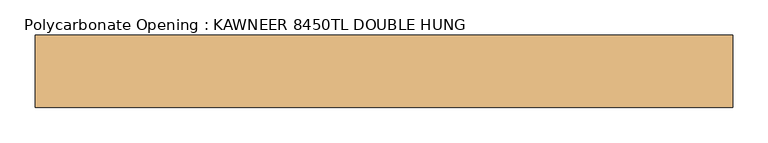
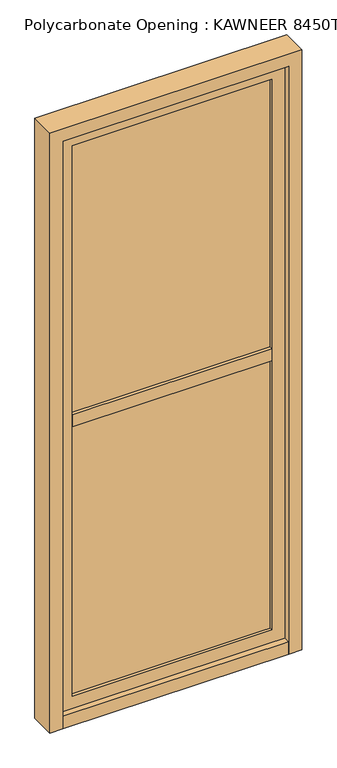
"""IFC4 building model written with IfcOpenShell, lengths in millimetres: door geometry, Polycarbonate Opening : KAWNEER 8450TL DOUBLE HUNG."""

from ifc_helpers import new_model, si_unit, frame, origin, origin_with_axes, place, context, project, spatial, polyline, outline, extrude, source, transform, mapped, element, save


def polycarbonate_opening_kawneer_8450tl_double_hung_34cef571(model_context):
    return source(origin(), model_context, "Body", "SweptSolid", [
        extrude(outline(polyline([(440.1908884, 12.7), (440.1908884, -12.7), (-440.1908884, -12.7), (-440.1908884, 12.7), (440.1908884, 12.7)])), frame((0.0, 0.0, 50.8), z_axis=(0.0, 0.0, 1.0), x_axis=(1.0, 0.0, 0.0)), (0.0, 0.0, 1.0), 2371.4648118),
        extrude(outline(polyline([(2422.2648118, -440.1908884), (0.0, -440.1908884), (0.0, 440.1908884), (2422.2648118, 440.1908884), (2422.2648118, -440.1908884)]), holes=[polyline([(101.6, 389.3908884), (101.6, -389.3908884), (2371.4648118, -389.3908884), (2371.4648118, 389.3908884), (101.6, 389.3908884)])]), frame((0.0, -25.4, 0.0), z_axis=(0.0, 1.0, 0.0), x_axis=(0.0, 0.0, 1.0)), (0.0, 0.0, 1.0), 50.8),
        extrude(outline(polyline([(2473.0648118, 490.9908884), (2473.0648118, -490.9908884), (0.0, -490.9908884), (0.0, -440.1908884), (2422.2648118, -440.1908884), (2422.2648118, 440.1908884), (0.0, 440.1908884), (0.0, 490.9908884), (2473.0648118, 490.9908884)])), frame((0.0, -50.8, 0.0), z_axis=(0.0, 1.0, 0.0), x_axis=(0.0, 0.0, 1.0)), (0.0, 0.0, 1.0), 101.6),
        extrude(outline(polyline([(440.1908884, 50.8), (440.1908884, -50.8), (-440.1908884, -50.8), (-440.1908884, 50.8), (440.1908884, 50.8)])), origin_with_axes(), (0.0, 0.0, 1.0), 50.8),
        extrude(outline(polyline([(389.3908884, 25.4), (389.3908884, -25.4), (-389.3908884, -25.4), (-389.3908884, 25.4), (389.3908884, 25.4)])), frame((0.0, 0.0, 1211.1324059), z_axis=(0.0, 0.0, 1.0), x_axis=(1.0, 0.0, 0.0)), (0.0, 0.0, 1.0), 50.8),
    ])


if __name__ == "__main__":
    model = new_model("IFC4")
    model_context = context("Model", 3, world=origin())
    ifc_project = project(units=[si_unit("LENGTHUNIT", "METRE", prefix="MILLI")], contexts=[model_context])
    site = spatial("IfcSite", under=ifc_project)
    building = spatial("IfcBuilding", under=site)
    placement = place(None, origin())
    polycarbonate_opening_kawneer_8450tl_double_hung_shape = polycarbonate_opening_kawneer_8450tl_double_hung_34cef571(model_context)
    element("IfcDoor", 1, ObjectType="Polycarbonate Opening : KAWNEER 8450TL DOUBLE HUNG", at=placement, inside=building, context=model_context, shape_type="MappedRepresentation", body=[
        mapped(polycarbonate_opening_kawneer_8450tl_double_hung_shape, transform((0.0, 0.0, 0.0), x_axis=(1.0, 0.0, 0.0), y_axis=(0.0, 1.0, 0.0), z_axis=(0.0, 0.0, 1.0))),
    ])
    save(model, "model.ifc")

# Revit data of these elements
# Type "Polycarbonate Opening : KAWNEER 8450TL DOUBLE HUNG"
#   Type Mark = "59"
#   OD_DS_Door_Material = "ALUM./GLAZING"
#   OD_DS_Door_Type = "STOREFRONT - DOUBLE HUNG WINDOW"
#   OD_DS_Lockset = "POLE OPERATOR HARDWARE FOR TOP SASH; BOTTOM SASH MECHANICALLY FIXED"
#   Analytic Construction = "<None>"
#   offset [instance default] = 0' - 2"
#   Stile = 0' - 2"
#   Mullion Width = 0' - 2"
#   Mullion Depth = 0' - 4"
#   Opening Size [instance default] = 5' - 1.50212"
#   Door Width [instance default] = 5' - 1.50212"
#   Window ON/OFF = no
#   Door On/Off = yes
#   Mullion Material = DOUBLE HUNG (CLEAR ANODIZED ALUM) - TEMPERED INSULATED GLAZING (CARDINAL GLASS LoĒ²-240\nOR EQUIVALENT)
#   Glass Material = TEMPERED INSULATED GLAZING (CARDINAL GLASS LoĒ²-240\nOR EQUIVALENT)
#   Door Material = DOUBLE HUNG (CLEAR ANODIZED ALUM) - TEMPERED INSULATED GLAZING (CARDINAL GLASS LoĒ²-240\nOR EQUIVALENT)
# Element 1 (IfcDoor, "Polycarbonate Opening : KAWNEER 8450TL DOUBLE HUNG")
#   offset = 0' - 0"
#   Materials on its faces: "DOUBLE HUNG (CLEAR ANODIZED ALUM) - TEMPERED INSULATED GLAZING (CARDINAL GLASS LoĒ²-240\nOR EQUIVALENT)", "TEMPERED INSULATED GLAZING (CARDINAL GLASS LoĒ²-240\nOR EQUIVALENT)"
# Materials
#   "DOUBLE HUNG (CLEAR ANODIZED ALUM) - TEMPERED INSULATED GLAZING (CARDINAL GLASS LoĒ²-240\nOR EQUIVALENT)": class "Metal", colour RGB 244 244 244, transparency 0, Description = "Aluminum 6061", Cost = 0
#   "TEMPERED INSULATED GLAZING (CARDINAL GLASS LoĒ²-240\nOR EQUIVALENT)": class "Glass", colour RGB 196 205 210, transparency 0.85, Description = "Soda Lime Glass", Cost = 0
